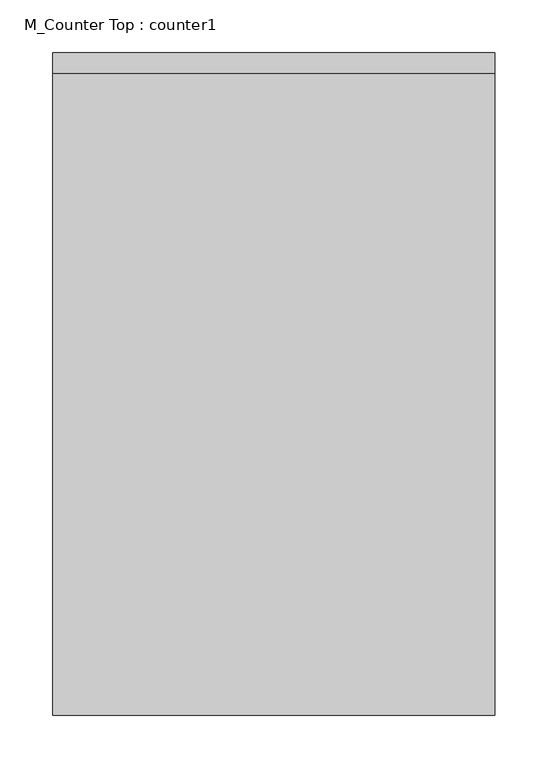
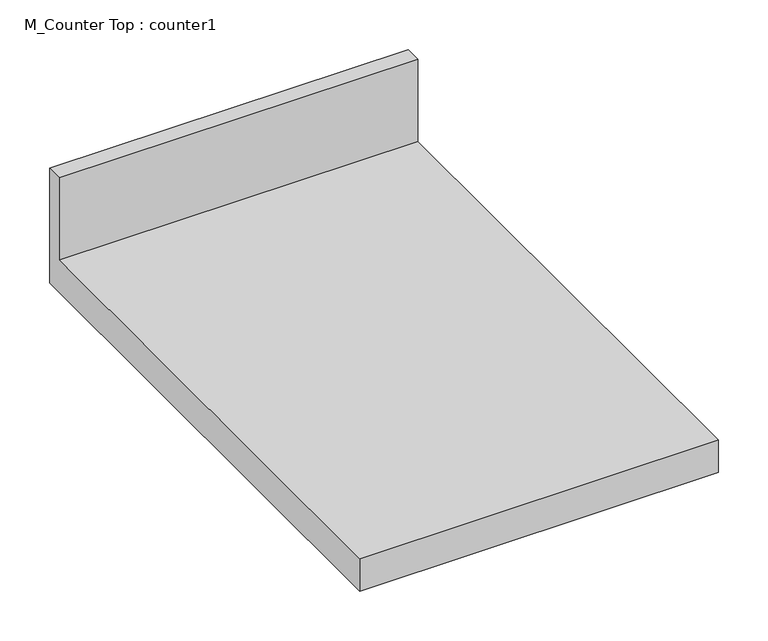
"""IFC4 building model written with IfcOpenShell, lengths in millimetres: furniture geometry, M_Counter Top : counter1."""

from ifc_helpers import new_model, si_unit, frame, origin, place, context, project, spatial, polyline, outline, extrude, source, transform, mapped, element, save


def m_counter_top_counter1_cb9ad101(model_context):
    return source(origin(), model_context, "Body", "SweptSolid", [
        extrude(outline(polyline([(0.0, 1001.6), (0.0, 860.0), (-625.0, 860.0), (-625.0, 900.0), (-19.05, 900.0), (-19.05, 1001.6), (0.0, 1001.6)])), frame((-1200.4622951, 0.0, 0.0), z_axis=(1.0, 0.0, 0.0), x_axis=(0.0, 1.0, 0.0)), (0.0, 0.0, 1.0), 417.1101467),
    ])


if __name__ == "__main__":
    model = new_model("IFC4")
    model_context = context("Model", 3, world=origin())
    ifc_project = project(units=[si_unit("LENGTHUNIT", "METRE", prefix="MILLI")], contexts=[model_context])
    site = spatial("IfcSite", under=ifc_project)
    building = spatial("IfcBuilding", under=site)
    placement = place(None, origin())
    m_counter_top_counter1_shape = m_counter_top_counter1_cb9ad101(model_context)
    element("IfcFurniture", 1, ObjectType="M_Counter Top : counter1", at=placement, inside=building, context=model_context, shape_type="MappedRepresentation", body=[
        mapped(m_counter_top_counter1_shape, transform((0.0, 0.0, 0.0), x_axis=(1.0, 0.0, 0.0), y_axis=(0.0, 1.0, 0.0), z_axis=(0.0, 0.0, 1.0))),
    ])
    save(model, "model.ifc")

# Revit data of these elements
# Type "M_Counter Top : counter1"
#   Counter Thickness = 0' - 1.5748"
#   Depth = 2' - 0.6063"
#   Height = 2' - 11.43307"
#   Length [instance default] = 8' - 2.4252"
#   Counter Top Material = Counter Top
#   Default Elevation = 0
# Element 1 (IfcFurniture, "M_Counter Top : counter1")
#   Length = 1' - 4.42166"
#   Materials on its faces: "Counter Top"
# Materials
#   "Counter Top": class "Wood", colour RGB 226 177 128, transparency 0
